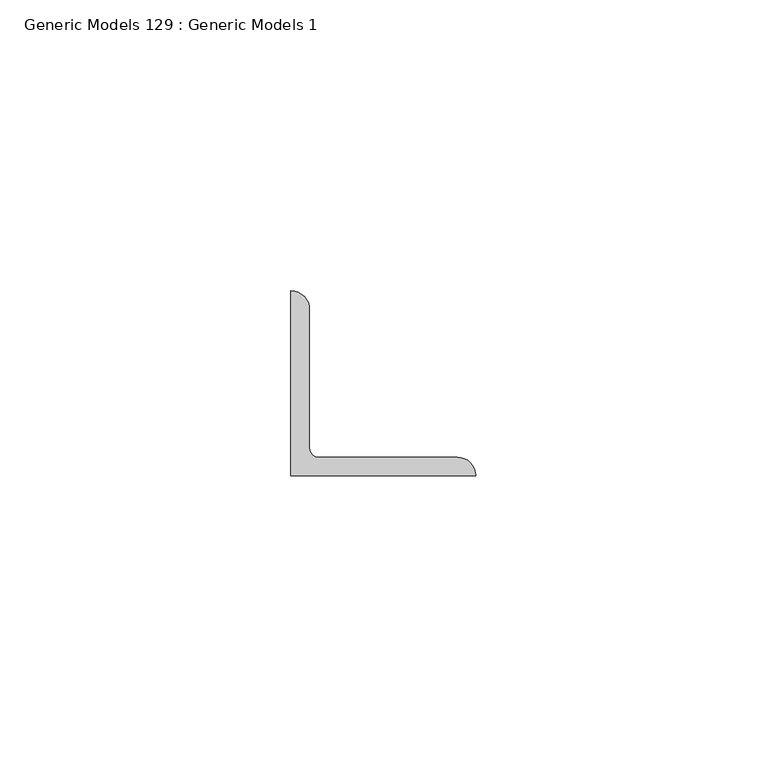
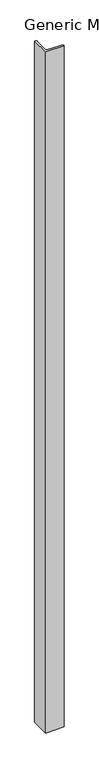
"""IFC4 building model written with IfcOpenShell, lengths in millimetres: proxy geometry, Generic Models 129 : Generic Models 1."""

from ifc_helpers import new_model, si_unit, point, frame, frame_2d, origin, place, context, project, spatial, polyline, circle_curve, trimmed, segment, composite_curve, outline, extrude, source, transform, mapped, element, save


def generic_models_129_generic_models_1_0c91dad2(model_context):
    return source(origin(), model_context, "Body", "SweptSolid", [
        extrude(outline(composite_curve([segment(polyline([(50229.5071108, -1305.9154992), (50229.5071108, -1274.1654992)]), True, "CONTINUOUS"), segment(trimmed(circle_curve(frame_2d((50229.5071108, -1277.3404992)), 3.175), [point((50229.5071108, -1274.1654992))], [point((50232.6821108, -1277.3404992))], False, "CARTESIAN"), True, "CONTINUOUS"), segment(polyline([(50232.6821108, -1277.3404992), (50232.6821108, -1301.1529992)]), True, "CONTINUOUS"), segment(trimmed(circle_curve(frame_2d((50234.2696108, -1301.1529992)), 1.5875), [point((50232.6821108, -1301.1529992))], [point((50234.2696108, -1302.7404992))], True, "CARTESIAN"), True, "CONTINUOUS"), segment(polyline([(50234.2696108, -1302.7404992), (50258.0821108, -1302.7404992)]), True, "CONTINUOUS"), segment(trimmed(circle_curve(frame_2d((50258.0821108, -1305.9154992)), 3.175), [point((50258.0821108, -1302.7404992))], [point((50261.2571108, -1305.9154992))], False, "CARTESIAN"), True, "CONTINUOUS"), segment(polyline([(50261.2571108, -1305.9154992), (50229.5071108, -1305.9154992)]), True, "CONTINUOUS")], self_intersect=False)), frame((0.0, 0.0, 3648.6681787), z_axis=(0.0, 0.0, 1.0), x_axis=(1.0, 0.0, 0.0)), (0.0, 0.0, 1.0), 1219.2),
    ])


if __name__ == "__main__":
    model = new_model("IFC4")
    model_context = context("Model", 3, world=origin())
    ifc_project = project(units=[si_unit("LENGTHUNIT", "METRE", prefix="MILLI")], contexts=[model_context])
    site = spatial("IfcSite", under=ifc_project)
    building = spatial("IfcBuilding", under=site)
    placement = place(None, origin())
    generic_models_129_generic_models_1_shape = generic_models_129_generic_models_1_0c91dad2(model_context)
    element("IfcBuildingElementProxy", 1, Name="Generic Models 129 : Generic Models 1", ObjectType="Generic Models 129 : Generic Models 1", at=placement, inside=building, context=model_context, shape_type="MappedRepresentation", body=[
        mapped(generic_models_129_generic_models_1_shape, transform((0.0, 0.0, 0.0), x_axis=(1.0, 0.0, 0.0), y_axis=(0.0, 1.0, 0.0), z_axis=(0.0, 0.0, 1.0))),
    ])
    save(model, "model.ifc")

# Revit data of these elements
# Element 1 (IfcBuildingElementProxy, "Generic Models 129 : Generic Models 1")
#   Materials on its faces: "BULKHEAD FRAME WORK"
# Materials
#   "BULKHEAD FRAME WORK": class "Metal", colour RGB 189 187 185, transparency 0, Description = "Structural steel 50ksi", Cost = 0
